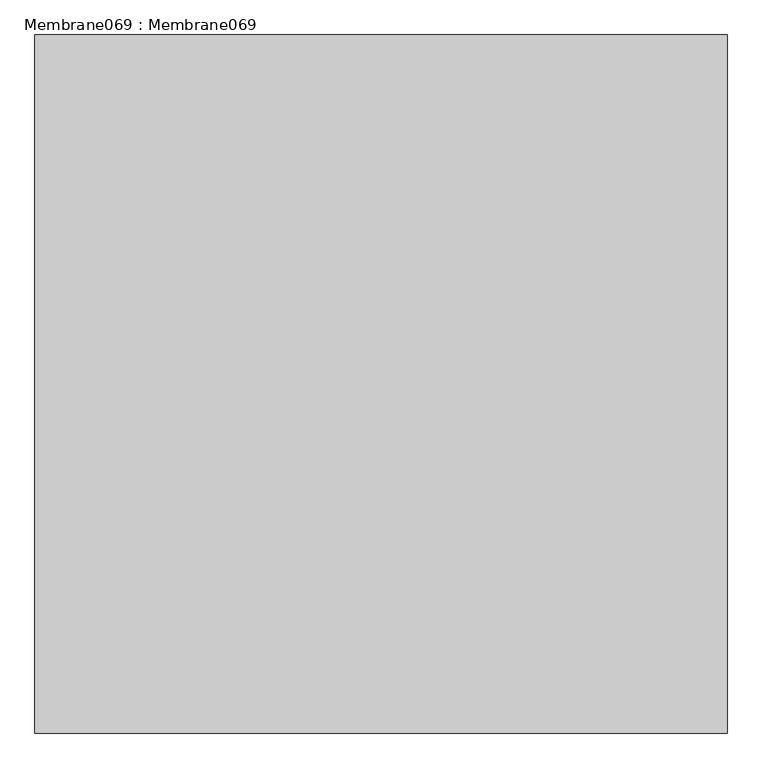
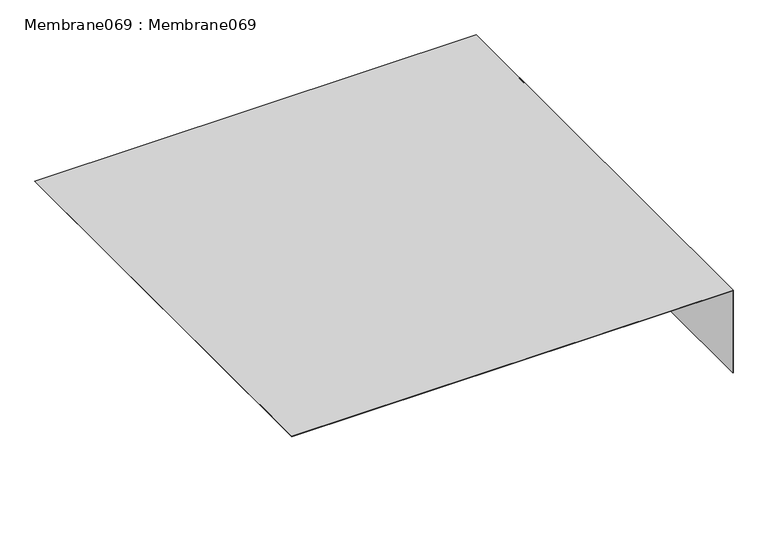
"""IFC4 building model written with IfcOpenShell, lengths in millimetres: proxy geometry, Membrane069 : Membrane069."""

from ifc_helpers import new_model, si_unit, frame, origin, place, context, project, spatial, polyline, outline, extrude, source, transform, mapped, element, save


def membrane069_membrane069_b3bdb6a2(model_context):
    return source(origin(), model_context, "Body", "SweptSolid", [
        extrude(outline(polyline([(43449.7282647, 15756.3258909), (43447.7282647, 15756.3258909), (43447.7282647, 17736.9891599), (43057.4548272, 17736.9891599), (43057.4548272, 17738.9891599), (43449.7282647, 17738.9891599), (43449.7282647, 15756.3258909)])), frame((0.0, 7982.1507711, 0.0), z_axis=(0.0, 1.0, 0.0), x_axis=(0.0, 0.0, 1.0)), (0.0, 0.0, 1.0), 2000.0),
    ])


if __name__ == "__main__":
    model = new_model("IFC4")
    model_context = context("Model", 3, world=origin())
    ifc_project = project(units=[si_unit("LENGTHUNIT", "METRE", prefix="MILLI")], contexts=[model_context])
    site = spatial("IfcSite", under=ifc_project)
    building = spatial("IfcBuilding", under=site)
    placement = place(None, origin())
    membrane069_membrane069_shape = membrane069_membrane069_b3bdb6a2(model_context)
    element("IfcBuildingElementProxy", 1, Name="Membrane069 : Membrane069", ObjectType="Membrane069 : Membrane069", at=placement, inside=building, context=model_context, shape_type="MappedRepresentation", body=[
        mapped(membrane069_membrane069_shape, transform((0.0, 0.0, 0.0), x_axis=(1.0, 0.0, 0.0), y_axis=(0.0, 1.0, 0.0), z_axis=(0.0, 0.0, 1.0))),
    ])
    save(model, "model.ifc")

# Revit data of these elements
# Type "Membrane069 : Membrane069"
#   NameOverride = "Membrane069"
# Element 1 (IfcBuildingElementProxy, "Membrane069 : Membrane069")
#   Materials on its faces: "(2) LAYERS OF ICE & WATER SHIELD (BITUTHANE) UNDER STUCCO"
# Materials
#   "(2) LAYERS OF ICE & WATER SHIELD (BITUTHANE) UNDER STUCCO": class "Unassigned", colour RGB 186 255 159, transparency 0, Cost = 0
